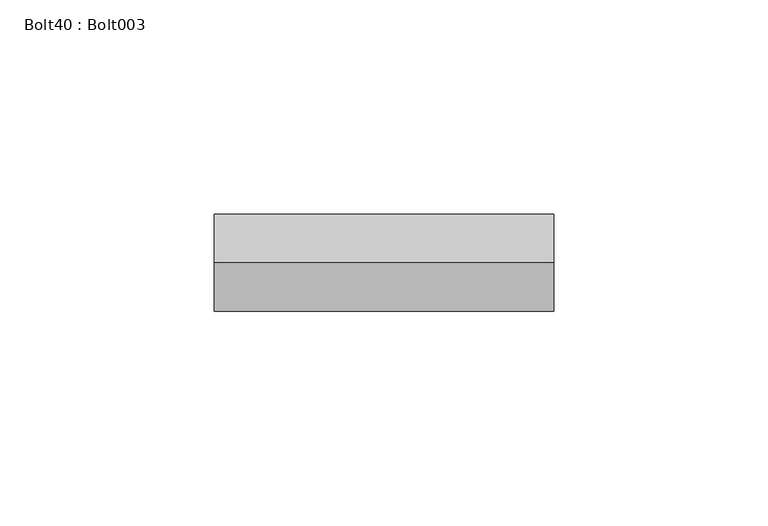
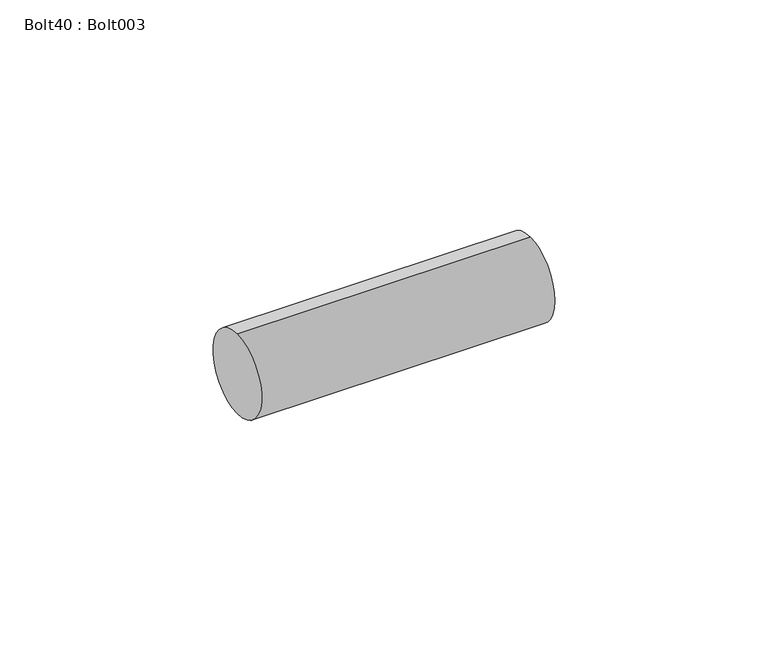
"""IFC4 building model written with IfcOpenShell, lengths in millimetres: proxy geometry, Bolt40 : Bolt003."""

from ifc_helpers import new_model, si_unit, point, frame, frame_2d, origin, place, context, project, spatial, circle_curve, trimmed, segment, composite_curve, outline, extrude, source, transform, mapped, element, save


def bolt40_bolt003_f55f5b75(model_context):
    return source(origin(), model_context, "Body", "SweptSolid", [
        extrude(outline(composite_curve([segment(trimmed(circle_curve(frame_2d((1985.8304801, 39960.0063132)), 11.4045168), [point((1985.8304801, 39971.41083))], [point((1985.8304801, 39948.6017964))], False, "CARTESIAN"), True, "CONTINUOUS"), segment(trimmed(circle_curve(frame_2d((1985.8304801, 39960.0063132)), 11.4045168), [point((1985.8304801, 39948.6017964))], [point((1985.8304801, 39971.41083))], False, "CARTESIAN"), True, "CONTINUOUS")], self_intersect=False)), frame((10265.0890809, 0.0, 0.0), z_axis=(1.0, 0.0, 0.0), x_axis=(0.0, 1.0, 0.0)), (0.0, 0.0, 1.0), 79.375),
    ])


if __name__ == "__main__":
    model = new_model("IFC4")
    model_context = context("Model", 3, world=origin())
    ifc_project = project(units=[si_unit("LENGTHUNIT", "METRE", prefix="MILLI")], contexts=[model_context])
    site = spatial("IfcSite", under=ifc_project)
    building = spatial("IfcBuilding", under=site)
    placement = place(None, origin())
    bolt40_bolt003_shape = bolt40_bolt003_f55f5b75(model_context)
    element("IfcBuildingElementProxy", 1, Name="Bolt40 : Bolt003", ObjectType="Bolt40 : Bolt003", at=placement, inside=building, context=model_context, shape_type="MappedRepresentation", body=[
        mapped(bolt40_bolt003_shape, transform((0.0, 0.0, 0.0), x_axis=(1.0, 0.0, 0.0), y_axis=(0.0, 1.0, 0.0), z_axis=(0.0, 0.0, 1.0))),
    ])
    save(model, "model.ifc")

# Revit data of these elements
# Type "Bolt40 : Bolt003"
#   NameOverride = "Bolt003"
# Element 1 (IfcBuildingElementProxy, "Bolt40 : Bolt003")
#   Materials on its faces: "STEEL ANGLE AND ANCHOR BOLT (SEE STRUCT. DWGS)"
# Materials
#   "STEEL ANGLE AND ANCHOR BOLT (SEE STRUCT. DWGS)": class "Unassigned", colour RGB 128 128 128, transparency 0, Cost = 0
